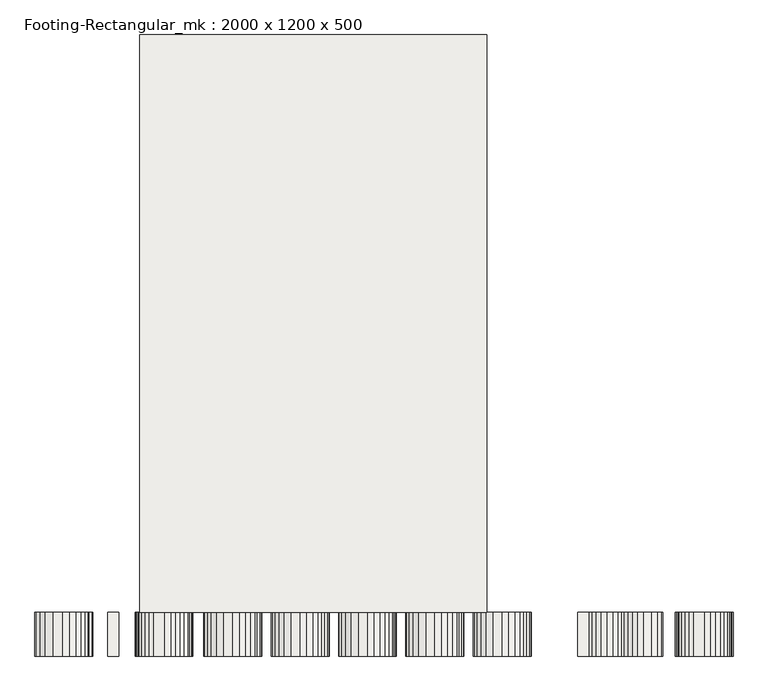
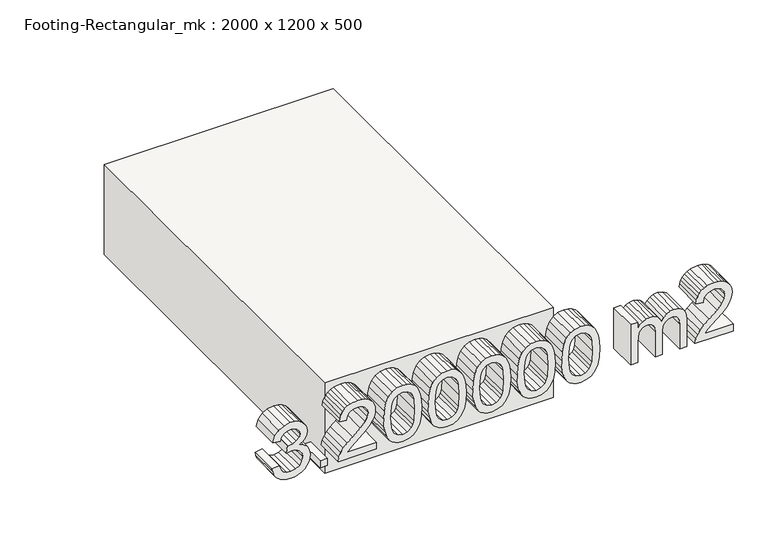
"""IFC4 building model written with IfcOpenShell, lengths in millimetres: slab geometry, Footing-Rectangular_mk : 2000 x 1200 x 500."""

from ifc_helpers import new_model, si_unit, frame, origin, place, context, project, spatial, polyline, outline, extrude, source, transform, mapped, element, save


def footing_rectangular_mk_2000_x_1200_x_500_fb34126d(model_context):
    return source(origin(), model_context, "Body", "SweptSolid", [
        extrude(outline(polyline([(600.0, 1085.6), (600.0, -914.4), (-600.0, -914.4), (-600.0, 1085.6), (600.0, 1085.6)])), frame((0.0, 0.0, -500.0), z_axis=(0.0, 0.0, 1.0), x_axis=(1.0, 0.0, 0.0)), (0.0, 0.0, 1.0), 500.0),
        extrude(outline(polyline([(-256.6091591, -963.6693211), (-274.6919009, -960.3836623), (-291.0179538, -954.2445459), (-305.5873178, -945.2519719), (-318.3999929, -933.4059404), (-328.8425323, -919.2780723), (-336.301489, -903.4399885), (-340.776863, -885.8916891), (-342.2686543, -866.6331742), (-340.5212601, -845.3251888), (-335.2790775, -825.9411961), (-326.5421064, -808.4811959), (-314.3103469, -792.9451883), (-299.5690318, -780.1929283), (-283.3033942, -771.0841713), (-265.5134339, -765.618917), (-246.199151, -763.7971656), (-218.947237, -767.4406684), (-196.6772554, -778.3711769), (-180.2814926, -796.0310121), (-170.6522351, -819.8624949), (-159.6659587, -801.719338), (-145.4451441, -788.6324706), (-128.7519525, -780.7134288), (-110.3485454, -778.0737481), (-90.5974139, -780.8528485), (-71.9430512, -789.1901496), (-55.7517708, -802.7789281), (-43.3898861, -821.3124603), (-35.5544961, -843.2943078), (-32.9426994, -867.2280318), (-38.24065, -900.4657005), (-54.1345016, -927.7547931), (-79.6576108, -947.7011122), (-113.8433338, -958.9104602), (-118.6021946, -920.8395735), (-97.7821784, -914.0916575), (-82.9107383, -902.1759161), (-73.9878742, -885.8545105), (-71.0135862, -865.8896022), (-73.9599903, -845.9618724), (-82.7992025, -830.0494314), (-96.1370254, -819.620834), (-112.5792614, -816.1446349), (-132.3210982, -820.9406743), (-146.1887161, -835.3287927), (-154.3865975, -855.721255), (-157.1192246, -878.5303263), (-156.6730814, -884.6276167), (-194.7439682, -888.8659772), (-190.5799649, -862.1717421), (-194.4744233, -838.2287235), (-206.1577985, -818.8958513), (-223.7897497, -806.1250021), (-245.5299362, -801.8680524), (-268.4319541, -806.1621807), (-287.318683, -819.0445657), (-299.9779965, -839.1953671), (-304.1977676, -865.2947445), (-301.1305331, -887.5368422), (-291.9288295, -904.5925251), (-275.7747276, -917.0752402), (-251.8502983, -925.5984343), (-256.6091591, -963.6693211)])), frame((0.0, -1066.8, 0.0), z_axis=(0.0, 1.0, 0.0), x_axis=(0.0, 0.0, 1.0)), (0.0, 0.0, 1.0), 152.4),
        extrude(outline(polyline([(-673.3788095, -1066.8), (-711.4496963, -1066.8), (-711.4496963, -914.4), (-673.3788095, -914.4), (-673.3788095, -1066.8)])), frame((0.0, 0.0, -337.5097935), z_axis=(0.0, 0.0, 1.0), x_axis=(1.0, 0.0, 0.0)), (0.0, 0.0, 1.0), 38.0708868),
        extrude(outline(polyline([(-299.4389067, -416.4003239), (-299.4389067, -565.9326545), (-280.068856, -548.7561412), (-243.4479346, -504.95975), (-214.1233136, -471.9172689), (-191.2863583, -450.4187432), (-172.1579684, -436.932206), (-153.9590436, -427.92569), (-136.0668422, -422.8508111), (-117.8586226, -421.1591848), (-100.5241002, -422.727657), (-84.6581325, -427.4330736), (-70.2607195, -435.2754346), (-57.3318613, -446.25474), (-46.661603, -459.9248466), (-39.0399899, -475.8396112), (-34.4670221, -493.9990338), (-32.9426994, -514.4031144), (-38.426543, -552.6877782), (-45.2813474, -568.5886008), (-54.8780736, -582.3284173), (-67.0865965, -593.6469774), (-81.776791, -602.284031), (-98.948657, -608.2395781), (-118.6021946, -611.5136186), (-123.3610555, -573.4427318), (-101.4814492, -569.3252018), (-84.9183827, -557.418755), (-74.4897853, -538.9688746), (-71.0135862, -515.2210437), (-74.5734372, -492.60716), (-85.2529901, -474.7335479), (-101.1003685, -463.1059406), (-120.1636959, -459.2300715), (-141.4298553, -463.3383069), (-163.2908723, -475.6630129), (-190.2267682, -500.3124249), (-226.7175645, -541.3947783), (-250.0192522, -569.1857821), (-270.8485631, -589.0577439), (-290.7484089, -602.7952368), (-311.2617017, -612.1828334), (-337.5097935, -616.2724794), (-337.5097935, -416.4003239), (-299.4389067, -416.4003239)])), frame((0.0, -1066.8, 0.0), z_axis=(0.0, 1.0, 0.0), x_axis=(0.0, 0.0, 1.0)), (0.0, 0.0, 1.0), 152.4),
        extrude(outline(polyline([(-187.6800341, -378.3294372), (-227.540141, -376.4333285), (-261.7583953, -370.7450027), (-290.334797, -361.2644596), (-313.2693461, -347.9916993), (-325.9565434, -334.1612599), (-335.0188273, -317.9513902), (-340.4561976, -299.36209), (-342.2686543, -278.3933594), (-338.0953565, -247.618773), (-325.5754628, -222.6626375), (-304.5695536, -203.3576493), (-274.9382091, -189.5365046), (-236.1516343, -181.2270874), (-187.6800341, -178.4572817), (-147.2947795, -180.1860866), (-116.1112284, -185.3725013), (-91.5547629, -193.2915432), (-71.0507648, -203.2182295), (-54.7386539, -216.3608647), (-42.7578499, -233.9277534), (-35.3964871, -254.9336626), (-32.9426994, -278.3933594), (-37.0881134, -309.0006422), (-49.5243552, -333.9010097), (-70.4466125, -353.2338819), (-100.0500731, -367.1386785), (-138.9295944, -375.5317475), (-187.6800341, -378.3294372)]), holes=[polyline([(-187.6056769, -340.2585504), (-128.4917023, -335.648404), (-107.1883643, -329.8857209), (-91.3874592, -321.8179646), (-76.1070544, -302.6709855), (-71.0135862, -278.8395026), (-76.7948585, -253.6695902), (-94.1386756, -233.779039), (-108.6522717, -226.2317831), (-129.0679706, -220.8408861), (-187.6056769, -216.5281684), (-247.3981609, -220.9896005), (-267.8765987, -226.5663905), (-282.0765004, -234.3738966), (-298.6674508, -254.3016264), (-304.1977676, -278.3933594), (-298.6860401, -302.4850924), (-282.1508576, -322.4128222), (-267.9741925, -330.2203283), (-247.4911074, -335.7971184), (-187.6056769, -340.2585504)])]), frame((0.0, -1066.8, 0.0), z_axis=(0.0, 1.0, 0.0), x_axis=(0.0, 0.0, 1.0)), (0.0, 0.0, 1.0), 152.4),
        extrude(outline(polyline([(-187.6800341, -145.1452558), (-227.540141, -143.2491471), (-261.7583953, -137.5608213), (-290.334797, -128.0802782), (-313.2693461, -114.8075179), (-325.9565434, -100.9770786), (-335.0188273, -84.7672088), (-340.4561976, -66.1779086), (-342.2686543, -45.209178), (-338.0953565, -14.4345916), (-325.5754628, 10.5215439), (-304.5695536, 29.8265321), (-274.9382091, 43.6476768), (-236.1516343, 51.957094), (-187.6800341, 54.7268997), (-147.2947795, 52.9980948), (-116.1112284, 47.8116801), (-91.5547629, 39.8926382), (-71.0507648, 29.9659519), (-54.7386539, 16.8233167), (-42.7578499, -0.743572), (-35.3964871, -21.7494812), (-32.9426994, -45.209178), (-37.0881134, -75.8164608), (-49.5243552, -100.7168283), (-70.4466125, -120.0497005), (-100.0500731, -133.9544971), (-138.9295944, -142.3475661), (-187.6800341, -145.1452558)]), holes=[polyline([(-187.6056769, -107.074369), (-128.4917023, -102.4642226), (-107.1883643, -96.7015395), (-91.3874592, -88.6337832), (-76.1070544, -69.4868041), (-71.0135862, -45.6553212), (-76.7948585, -20.4854088), (-94.1386756, -0.5948576), (-108.6522717, 6.9523983), (-129.0679706, 12.3432953), (-187.6056769, 16.656013), (-247.3981609, 12.1945809), (-267.8765987, 6.6177909), (-282.0765004, -1.1897152), (-298.6674508, -21.117445), (-304.1977676, -45.209178), (-298.6860401, -69.3009111), (-282.1508576, -89.2286408), (-267.9741925, -97.0361469), (-247.4911074, -102.612937), (-187.6056769, -107.074369)])]), frame((0.0, -1066.8, 0.0), z_axis=(0.0, 1.0, 0.0), x_axis=(0.0, 0.0, 1.0)), (0.0, 0.0, 1.0), 152.4),
        extrude(outline(polyline([(-187.6800341, 88.0389256), (-227.540141, 89.9350342), (-261.7583953, 95.6233601), (-290.334797, 105.1039032), (-313.2693461, 118.3766635), (-325.9565434, 132.2071028), (-335.0188273, 148.4169726), (-340.4561976, 167.0062728), (-342.2686543, 187.9750034), (-338.0953565, 218.7495898), (-325.5754628, 243.7057253), (-304.5695536, 263.0107135), (-274.9382091, 276.8318582), (-236.1516343, 285.1412754), (-187.6800341, 287.9110811), (-147.2947795, 286.1822762), (-116.1112284, 280.9958614), (-91.5547629, 273.0768196), (-71.0507648, 263.1501333), (-54.7386539, 250.0074981), (-42.7578499, 232.4406094), (-35.3964871, 211.4347002), (-32.9426994, 187.9750034), (-37.0881134, 157.3677206), (-49.5243552, 132.467353), (-70.4466125, 113.1344809), (-100.0500731, 99.2296843), (-138.9295944, 90.8366153), (-187.6800341, 88.0389256)]), holes=[polyline([(-187.6056769, 126.1098124), (-128.4917023, 130.7199588), (-107.1883643, 136.4826419), (-91.3874592, 144.5503982), (-76.1070544, 163.6973773), (-71.0135862, 187.5288602), (-76.7948585, 212.6987726), (-94.1386756, 232.5893238), (-108.6522717, 240.1365797), (-129.0679706, 245.5274767), (-187.6056769, 249.8401944), (-247.3981609, 245.3787623), (-267.8765987, 239.8019723), (-282.0765004, 231.9944662), (-298.6674508, 212.0667364), (-304.1977676, 187.9750034), (-298.6860401, 163.8832703), (-282.1508576, 143.9555406), (-267.9741925, 136.1480345), (-247.4911074, 130.5712444), (-187.6056769, 126.1098124)])]), frame((0.0, -1066.8, 0.0), z_axis=(0.0, 1.0, 0.0), x_axis=(0.0, 0.0, 1.0)), (0.0, 0.0, 1.0), 152.4),
        extrude(outline(polyline([(-187.6800341, 321.223107), (-227.540141, 323.1192156), (-261.7583953, 328.8075415), (-290.334797, 338.2880846), (-313.2693461, 351.5608449), (-325.9565434, 365.3912842), (-335.0188273, 381.601154), (-340.4561976, 400.1904542), (-342.2686543, 421.1591848), (-338.0953565, 451.9337712), (-325.5754628, 476.8899067), (-304.5695536, 496.1948949), (-274.9382091, 510.0160396), (-236.1516343, 518.3254568), (-187.6800341, 521.0952625), (-147.2947795, 519.3664576), (-116.1112284, 514.1800428), (-91.5547629, 506.261001), (-71.0507648, 496.3343147), (-54.7386539, 483.1916795), (-42.7578499, 465.6247908), (-35.3964871, 444.6188816), (-32.9426994, 421.1591848), (-37.0881134, 390.551902), (-49.5243552, 365.6515344), (-70.4466125, 346.3186623), (-100.0500731, 332.4138657), (-138.9295944, 324.0207967), (-187.6800341, 321.223107)]), holes=[polyline([(-187.6056769, 359.2939938), (-128.4917023, 363.9041402), (-107.1883643, 369.6668233), (-91.3874592, 377.7345796), (-76.1070544, 396.8815587), (-71.0135862, 420.7130416), (-76.7948585, 445.882954), (-94.1386756, 465.7735052), (-108.6522717, 473.3207611), (-129.0679706, 478.7116581), (-187.6056769, 483.0243757), (-247.3981609, 478.5629437), (-267.8765987, 472.9861537), (-282.0765004, 465.1786476), (-298.6674508, 445.2509178), (-304.1977676, 421.1591848), (-298.6860401, 397.0674517), (-282.1508576, 377.139722), (-267.9741925, 369.3322159), (-247.4911074, 363.7554258), (-187.6056769, 359.2939938)])]), frame((0.0, -1066.8, 0.0), z_axis=(0.0, 1.0, 0.0), x_axis=(0.0, 0.0, 1.0)), (0.0, 0.0, 1.0), 152.4),
        extrude(outline(polyline([(-187.6800341, 554.4072884), (-227.540141, 556.303397), (-261.7583953, 561.9917229), (-290.334797, 571.472266), (-313.2693461, 584.7450263), (-325.9565434, 598.5754656), (-335.0188273, 614.7853354), (-340.4561976, 633.3746356), (-342.2686543, 654.3433662), (-338.0953565, 685.1179526), (-325.5754628, 710.0740881), (-304.5695536, 729.3790763), (-274.9382091, 743.200221), (-236.1516343, 751.5096382), (-187.6800341, 754.2794439), (-147.2947795, 752.550639), (-116.1112284, 747.3642242), (-91.5547629, 739.4451824), (-71.0507648, 729.5184961), (-54.7386539, 716.3758608), (-42.7578499, 698.8089722), (-35.3964871, 677.803063), (-32.9426994, 654.3433662), (-37.0881134, 623.7360834), (-49.5243552, 598.8357158), (-70.4466125, 579.5028437), (-100.0500731, 565.5980471), (-138.9295944, 557.2049781), (-187.6800341, 554.4072884)]), holes=[polyline([(-187.6056769, 592.4781752), (-128.4917023, 597.0883216), (-107.1883643, 602.8510047), (-91.3874592, 610.918761), (-76.1070544, 630.0657401), (-71.0135862, 653.897223), (-76.7948585, 679.0671354), (-94.1386756, 698.9576866), (-108.6522717, 706.5049425), (-129.0679706, 711.8958395), (-187.6056769, 716.2085571), (-247.3981609, 711.7471251), (-267.8765987, 706.1703351), (-282.0765004, 698.362829), (-298.6674508, 678.4350992), (-304.1977676, 654.3433662), (-298.6860401, 630.2516331), (-282.1508576, 610.3239033), (-267.9741925, 602.5163973), (-247.4911074, 596.9396072), (-187.6056769, 592.4781752)])]), frame((0.0, -1066.8, 0.0), z_axis=(0.0, 1.0, 0.0), x_axis=(0.0, 0.0, 1.0)), (0.0, 0.0, 1.0), 152.4),
        extrude(outline(polyline([(-337.5097935, 916.0807126), (-337.5097935, 954.1515994), (-224.70992, 954.1515994), (-198.5175961, 955.6015648), (-179.2776704, 959.951461), (-165.4100525, 967.5358955), (-155.3346518, 978.6894756), (-149.2001827, 992.2038968), (-147.1553597, 1006.8708547), (-150.2225942, 1024.1310199), (-159.4242978, 1035.7586272), (-174.7790598, 1042.3671234), (-196.3054694, 1044.5699554), (-337.5097935, 1044.5699554), (-337.5097935, 1082.6408422), (-211.2512667, 1082.6408422), (-182.2333691, 1086.3679969), (-162.3985859, 1097.5494609), (-150.9661662, 1114.3634829), (-147.1553597, 1134.9883115), (-148.6425037, 1146.6716866), (-153.1039358, 1156.7377927), (-159.9912715, 1164.5638881), (-168.7561265, 1169.5272312), (-200.5438298, 1173.0591982), (-337.5097935, 1173.0591982), (-337.5097935, 1211.130085), (-184.1852457, 1211.130085), (-150.8639251, 1206.7708941), (-127.4878801, 1193.6933214), (-113.6853247, 1172.5294032), (-109.084473, 1143.9111756), (-111.8496314, 1124.1786334), (-120.1451066, 1106.3979678), (-133.9708986, 1090.5691787), (-153.3270074, 1076.6922661), (-134.6912339, 1068.4014383), (-120.7213749, 1055.7235355), (-111.9936984, 1038.7515045), (-109.084473, 1017.5782916), (-111.9379305, 997.8178655), (-120.4983033, 980.325334), (-133.7431796, 965.6026083), (-150.6501481, 954.1515994), (-113.8433338, 954.1515994), (-113.8433338, 916.0807126), (-337.5097935, 916.0807126)])), frame((0.0, -1066.8, 0.0), z_axis=(0.0, 1.0, 0.0), x_axis=(0.0, 0.0, 1.0)), (0.0, 0.0, 1.0), 152.4),
        extrude(outline(polyline([(-299.4389067, 1453.8319881), (-299.4389067, 1304.2996575), (-280.068856, 1321.4761708), (-243.4479346, 1365.2725621), (-214.1233136, 1398.3150431), (-191.2863583, 1419.8135688), (-172.1579684, 1433.300106), (-153.9590436, 1442.306622), (-136.0668422, 1447.3815009), (-117.8586226, 1449.0731272), (-100.5241002, 1447.504655), (-84.6581325, 1442.7992384), (-70.2607195, 1434.9568774), (-57.3318613, 1423.977572), (-46.661603, 1410.3074654), (-39.0399899, 1394.3927008), (-34.4670221, 1376.2332782), (-32.9426994, 1355.8291976), (-38.426543, 1317.5445339), (-45.2813474, 1301.6437112), (-54.8780736, 1287.9038947), (-67.0865965, 1276.5853346), (-81.776791, 1267.948281), (-98.948657, 1261.9927339), (-118.6021946, 1258.7186935), (-123.3610555, 1296.7895802), (-101.4814492, 1300.9071102), (-84.9183827, 1312.813557), (-74.4897853, 1331.2634374), (-71.0135862, 1355.0112684), (-74.5734372, 1377.625152), (-85.2529901, 1395.4987641), (-101.1003685, 1407.1263714), (-120.1636959, 1411.0022405), (-141.4298553, 1406.8940051), (-163.2908723, 1394.5692991), (-190.2267682, 1369.9198871), (-226.7175645, 1328.8375337), (-250.0192522, 1301.04653), (-270.8485631, 1281.1745681), (-290.7484089, 1267.4370752), (-311.2617017, 1258.0494786), (-337.5097935, 1253.9598326), (-337.5097935, 1453.8319881), (-299.4389067, 1453.8319881)])), frame((0.0, -1066.8, 0.0), z_axis=(0.0, 1.0, 0.0), x_axis=(0.0, 0.0, 1.0)), (0.0, 0.0, 1.0), 152.4),
    ])


if __name__ == "__main__":
    model = new_model("IFC4")
    model_context = context("Model", 3, world=origin())
    ifc_project = project(units=[si_unit("LENGTHUNIT", "METRE", prefix="MILLI")], contexts=[model_context])
    site = spatial("IfcSite", under=ifc_project)
    building = spatial("IfcBuilding", under=site)
    placement = place(None, origin())
    footing_rectangular_mk_2000_x_1200_x_500_shape = footing_rectangular_mk_2000_x_1200_x_500_fb34126d(model_context)
    element("IfcSlab", 1, ObjectType="Footing-Rectangular_mk : 2000 x 1200 x 500", at=placement, inside=building, context=model_context, shape_type="MappedRepresentation", body=[
        mapped(footing_rectangular_mk_2000_x_1200_x_500_shape, transform((0.0, 0.0, 0.0), x_axis=(1.0, 0.0, 0.0), y_axis=(0.0, 1.0, 0.0), z_axis=(0.0, 0.0, 1.0))),
    ])
    save(model, "model.ifc")

# Revit data of these elements
# Type "Footing-Rectangular_mk : 2000 x 1200 x 500"
#   ModelText [instance default] = "ModelText"
#   Assembly Code = "A1010100"
#   Width = 1200 mm
#   Length = 2000 mm
#   Foundation Thickness = 500 mm
#   Structural Material [instance default] = Concrete, Cast-in-Place gray
# Element 1 (IfcSlab, "Footing-Rectangular_mk : 2000 x 1200 x 500")
#   ModelText = "3.200000 m2"
#   Materials on its faces: "Concrete, Cast-in-Place gray"
# Materials
#   "Concrete, Cast-in-Place gray": class "Concrete", colour RGB 192 192 192, transparency 0, Description = "Cast-in-place concrete", Cost = 0
